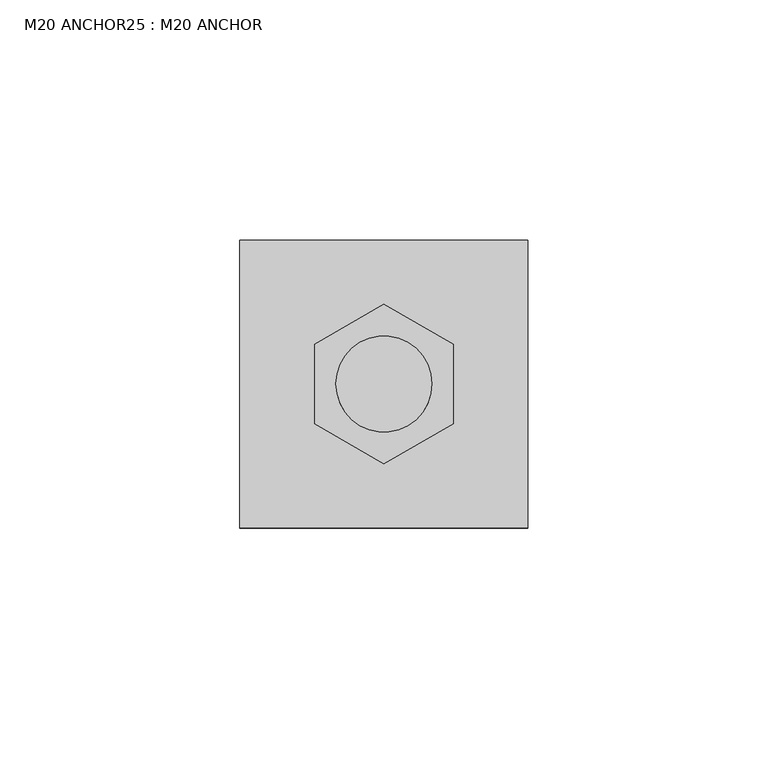
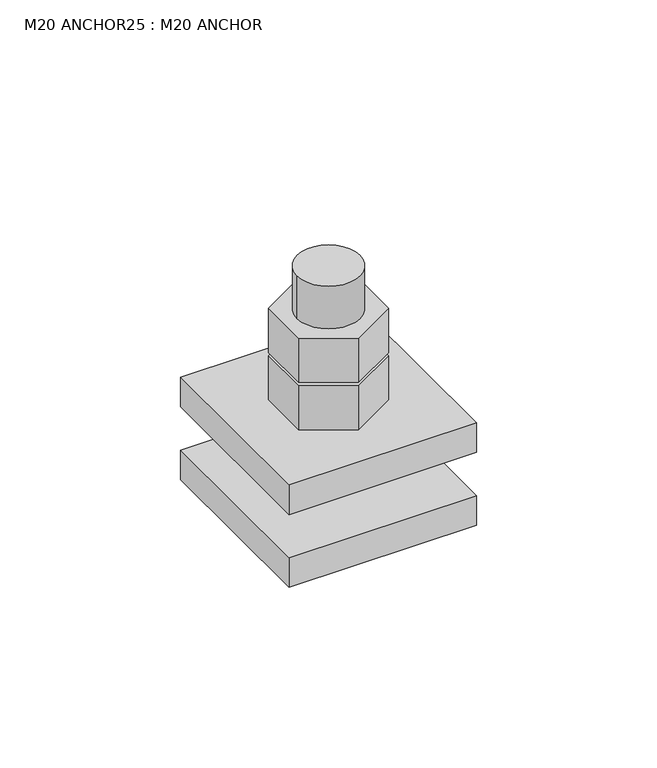
"""IFC4 building model written with IfcOpenShell, lengths in millimetres: fastener geometry, M20 ANCHOR25 : M20 ANCHOR."""

import ifcopenshell
import ifcopenshell.guid

model = None  # the IFC model being written
_history = None  # IfcOwnerHistory: only IFC2X3 demands one
_inside = {}  # id of a spatial element -> (the spatial element, [elements in it])
_under = {}  # id of a project, library or spatial element -> (it, [spatial elements below it])
_declared = {}  # id of a project -> (the project, [libraries it declares])
_typed = {}  # id of a type object -> (the type object, [elements of that type])
_made_of = {}  # id of a material, layer set ... -> (it, [elements and type objects made of it])


def new_model(schema):
    """Start an empty IFC model of exactly this schema.

    Asked for "IFC4X3", IfcOpenShell would pick the latest addendum, in which some entities
    have other attributes; the version numbers below select the first issue.
    IFC2X3 requires an IfcOwnerHistory on every rooted entity: one is made here for all.
    """
    global model, _history
    if schema == "IFC4X3":
        model = ifcopenshell.file(schema_version=(4, 3, 0, 0))
    else:
        model = ifcopenshell.file(schema=schema)
    _inside.clear()
    _under.clear()
    _declared.clear()
    _typed.clear()
    _made_of.clear()
    _history = None
    if model.schema == "IFC2X3":
        org = make("IfcOrganization", Name="unknown")
        user = make(
            "IfcPersonAndOrganization",
            ThePerson=make("IfcPerson", FamilyName="unknown"),
            TheOrganization=org,
        )
        app = make(
            "IfcApplication",
            ApplicationDeveloper=org,
            Version="unknown",
            ApplicationFullName="unknown",
            ApplicationIdentifier="unknown",
        )
        _history = make(
            "IfcOwnerHistory",
            OwningUser=user,
            OwningApplication=app,
            ChangeAction="ADDED",
            CreationDate=0,
        )
    return model


def make(cls, **values):
    """One entity of the class cls with the attributes given. An attribute that is None is left unset."""
    return model.create_entity(
        cls, **{name: value for name, value in values.items() if value is not None}
    )


def rooted(cls, **values):
    """An entity with a GlobalId (a new one), such as an element, a storey or a relation."""
    return make(cls, GlobalId=ifcopenshell.guid.new(), OwnerHistory=_history, **values)


def si_unit(unit_type, name, prefix=None):
    """IfcSIUnit, for example si_unit("LENGTHUNIT", "METRE", prefix="MILLI")."""
    return make("IfcSIUnit", UnitType=unit_type, Prefix=prefix, Name=name)


def assignment(units):
    """IfcUnitAssignment: the units of a project."""
    return None if units is None else make("IfcUnitAssignment", Units=units)


def point(xyz):
    """IfcCartesianPoint."""
    return None if xyz is None else make("IfcCartesianPoint", Coordinates=xyz)


def direction(xyz):
    """IfcDirection."""
    return None if xyz is None else make("IfcDirection", DirectionRatios=xyz)


def frame(location, z_axis=None, x_axis=None):
    """IfcAxis2Placement3D, a coordinate frame: its origin and axes. An axis left out is left unset."""
    return make(
        "IfcAxis2Placement3D",
        Location=point(location),
        Axis=direction(z_axis),
        RefDirection=direction(x_axis),
    )


def frame_2d(location, x_axis=None):
    """IfcAxis2Placement2D, a coordinate frame in the plane: its origin and x axis."""
    return make(
        "IfcAxis2Placement2D", Location=point(location), RefDirection=direction(x_axis)
    )


def origin():
    """The frame at (0, 0, 0) with its axes left unset."""
    return frame((0.0, 0.0, 0.0))


def place(relative_to, where):
    """IfcLocalPlacement: puts the frame where relative to a parent placement (None: the world)."""
    return make(
        "IfcLocalPlacement", PlacementRelTo=relative_to, RelativePlacement=where
    )


def context(
    kind, dimensions, precision=None, world=None, true_north=None, identifier=None
):
    """IfcGeometricRepresentationContext, for example the 3D "Model" context."""
    return make(
        "IfcGeometricRepresentationContext",
        ContextIdentifier=identifier,
        ContextType=kind,
        CoordinateSpaceDimension=dimensions,
        Precision=precision,
        WorldCoordinateSystem=world,
        TrueNorth=true_north,
    )


def project(units=None, contexts=None):
    """IfcProject with its units and contexts."""
    return rooted(
        "IfcProject",
        Name="project",
        RepresentationContexts=contexts,
        UnitsInContext=assignment(units),
    )


def spatial(cls, under=None, at=None, **own):
    """A site, building, storey or space (cls), placed at a placement, below another one or the project."""
    s = rooted(cls, ObjectPlacement=at, **own)
    if under is not None:
        _under.setdefault(under.id(), (under, []))[1].append(s)
    return s


def polyline(points):
    """IfcPolyline through the points."""
    return make("IfcPolyline", Points=[point(p) for p in points])


def circle_curve(where, radius):
    """IfcCircle in the frame where."""
    return make("IfcCircle", Position=where, Radius=radius)


def trimmed(basis, trim1, trim2, sense, master):
    """IfcTrimmedCurve: the piece of a basis curve between two trims."""
    return make(
        "IfcTrimmedCurve",
        BasisCurve=basis,
        Trim1=trim1,
        Trim2=trim2,
        SenseAgreement=sense,
        MasterRepresentation=master,
    )


def segment(curve, same_sense, transition):
    """IfcCompositeCurveSegment."""
    return make(
        "IfcCompositeCurveSegment",
        Transition=transition,
        SameSense=same_sense,
        ParentCurve=curve,
    )


def composite_curve(segments, self_intersect=None):
    """IfcCompositeCurve: segments joined end to end."""
    return make("IfcCompositeCurve", Segments=segments, SelfIntersect=self_intersect)


def outline(outer, holes=None, kind="AREA"):
    """IfcArbitraryClosedProfileDef: a profile drawn as a closed curve; with holes, ...WithVoids."""
    if holes is None:
        return make("IfcArbitraryClosedProfileDef", ProfileType=kind, OuterCurve=outer)
    return make(
        "IfcArbitraryProfileDefWithVoids",
        ProfileType=kind,
        OuterCurve=outer,
        InnerCurves=holes,
    )


def extrude(swept, where, along, depth):
    """IfcExtrudedAreaSolid: the profile swept, set in the frame where, extruded along a direction by depth."""
    return make(
        "IfcExtrudedAreaSolid",
        SweptArea=swept,
        Position=where,
        ExtrudedDirection=direction(along),
        Depth=depth,
    )


def shape(context_of_items, identifier, shape_type, items):
    """IfcShapeRepresentation: the items that make up one representation, for example the "Body"."""
    return make(
        "IfcShapeRepresentation",
        ContextOfItems=context_of_items,
        RepresentationIdentifier=identifier,
        RepresentationType=shape_type,
        Items=items,
    )


def source(mapping_origin, context_of_items, identifier, shape_type, items):
    """IfcRepresentationMap: a shape defined once, which mapped items show again and again."""
    return make(
        "IfcRepresentationMap",
        MappingOrigin=mapping_origin,
        MappedRepresentation=shape(context_of_items, identifier, shape_type, items),
    )


def transform(
    local_origin,
    x_axis=None,
    y_axis=None,
    z_axis=None,
    scale=None,
    scale2=None,
    scale3=None,
    uniform=True,
):
    """IfcCartesianTransformationOperator3D, or its non-uniform kind. x_axis, y_axis, z_axis: its Axis1, 2, 3."""
    if uniform:
        return make(
            "IfcCartesianTransformationOperator3D",
            Axis1=direction(x_axis),
            Axis2=direction(y_axis),
            LocalOrigin=point(local_origin),
            Scale=scale,
            Axis3=direction(z_axis),
        )
    return make(
        "IfcCartesianTransformationOperator3DnonUniform",
        Axis1=direction(x_axis),
        Axis2=direction(y_axis),
        LocalOrigin=point(local_origin),
        Scale=scale,
        Axis3=direction(z_axis),
        Scale2=scale2,
        Scale3=scale3,
    )


def mapped(mapping_source, mapping_target):
    """IfcMappedItem: shows the shape of a source again, moved by a transform."""
    return make(
        "IfcMappedItem", MappingSource=mapping_source, MappingTarget=mapping_target
    )


def made_of(thing, what):
    """Note that an element or type object is made of a material, layer set ...; save() writes the relation."""
    if what is not None:
        _made_of.setdefault(what.id(), (what, []))[1].append(thing)
    return thing


def element(
    cls,
    number,
    at=None,
    inside=None,
    cuts=None,
    type_object=None,
    material=None,
    context=None,
    identifier="Body",
    shape_type=None,
    held_by="IfcProductDefinitionShape",
    body=None,
    shapes=None,
    **own,
):
    """One element of the class cls, such as IfcWall. Its Tag is "e" and its number.

    at: its placement. inside: the storey or other place that contains it. cuts: it is an
    opening in that element (IfcRelVoidsElement). A single representation is given by context,
    identifier, shape_type and body (its items); several are given by shapes. held_by: the class
    of the entity that holds the representations. save() writes the other relations.
    """
    e = rooted(cls, Tag="e%d" % number, ObjectPlacement=at, **own)
    if body is not None:
        shapes = [shape(context, identifier, shape_type, body)]
    if shapes is not None:
        e.Representation = make(held_by, Representations=shapes)
    if inside is not None:
        _inside.setdefault(inside.id(), (inside, []))[1].append(e)
    if cuts is not None:
        rooted(
            "IfcRelVoidsElement", RelatingBuildingElement=cuts, RelatedOpeningElement=e
        )
    if type_object is not None:
        _typed.setdefault(type_object.id(), (type_object, []))[1].append(e)
    return made_of(e, material)


def aggregate(whole, parts):
    """IfcRelAggregates: a whole, such as a stair, and the parts it consists of."""
    return rooted("IfcRelAggregates", RelatingObject=whole, RelatedObjects=parts)


def save(model, path):
    """Write the relations noted so far, then the file.

    IfcRelAggregates (storeys below a building ...), IfcRelContainedInSpatialStructure (elements
    in a storey), IfcRelDefinesByType, IfcRelAssociatesMaterial and IfcRelDeclares: one each for
    every whole, place, type object, material and project.
    """
    for whole, parts in _under.values():
        aggregate(whole, parts)
    for where, things in _inside.values():
        rooted(
            "IfcRelContainedInSpatialStructure",
            RelatedElements=things,
            RelatingStructure=where,
        )
    for kind, things in _typed.values():
        rooted("IfcRelDefinesByType", RelatedObjects=things, RelatingType=kind)
    for what, things in _made_of.values():
        rooted("IfcRelAssociatesMaterial", RelatedObjects=things, RelatingMaterial=what)
    for by, libraries in _declared.values():
        rooted("IfcRelDeclares", RelatingContext=by, RelatedDefinitions=libraries)
    model.write(path)


def m20_anchor25_m20_anchor_22db5d31(model_context):
    return source(origin(), model_context, "Body", "SweptSolid", [
        extrude(outline(polyline([(-30872.0439916, -7533.2988347), (-30886.4521106, -7541.6173661), (-30900.8602297, -7533.2988347), (-30900.8602297, -7516.6617719), (-30886.4521106, -7508.3432405), (-30872.0439916, -7516.6617719), (-30872.0439916, -7533.2988347)]), holes=[composite_curve([segment(trimmed(circle_curve(frame_2d((-30886.4521106, -7524.9803033)), 10.0), [point((-30896.4521106, -7524.9803033))], [point((-30876.4521106, -7524.9803033))], True, "CARTESIAN"), True, "CONTINUOUS"), segment(trimmed(circle_curve(frame_2d((-30886.4521106, -7524.9803033)), 10.0), [point((-30876.4521106, -7524.9803033))], [point((-30896.4521106, -7524.9803033))], True, "CARTESIAN"), True, "CONTINUOUS")], self_intersect=False)]), frame((0.0, 0.0, 240.6), z_axis=(0.0, 0.0, 1.0), x_axis=(1.0, 0.0, 0.0)), (0.0, 0.0, 1.0), 15.0),
        extrude(outline(polyline([(-30872.0439916, -7533.2988347), (-30886.4521106, -7541.6173661), (-30900.8602297, -7533.2988347), (-30900.8602297, -7516.6617719), (-30886.4521106, -7508.3432405), (-30872.0439916, -7516.6617719), (-30872.0439916, -7533.2988347)]), holes=[composite_curve([segment(trimmed(circle_curve(frame_2d((-30886.4521106, -7524.9803033)), 10.0), [point((-30896.4521106, -7524.9803033))], [point((-30876.4521106, -7524.9803033))], True, "CARTESIAN"), True, "CONTINUOUS"), segment(trimmed(circle_curve(frame_2d((-30886.4521106, -7524.9803033)), 10.0), [point((-30876.4521106, -7524.9803033))], [point((-30896.4521106, -7524.9803033))], True, "CARTESIAN"), True, "CONTINUOUS")], self_intersect=False)]), frame((0.0, 0.0, 224.6), z_axis=(0.0, 0.0, 1.0), x_axis=(1.0, 0.0, 0.0)), (0.0, 0.0, 1.0), 15.0),
        extrude(outline(composite_curve([segment(trimmed(circle_curve(frame_2d((-30886.4521106, -7524.9803033)), 10.0), [point((-30896.4521106, -7524.9803033))], [point((-30876.4521106, -7524.9803033))], False, "CARTESIAN"), True, "CONTINUOUS"), segment(trimmed(circle_curve(frame_2d((-30886.4521106, -7524.9803033)), 10.0), [point((-30876.4521106, -7524.9803033))], [point((-30896.4521106, -7524.9803033))], False, "CARTESIAN"), True, "CONTINUOUS")], self_intersect=False)), frame((0.0, 0.0, 190.0), z_axis=(0.0, 0.0, 1.0), x_axis=(1.0, 0.0, 0.0)), (0.0, 0.0, 1.0), 80.0),
        extrude(outline(polyline([(-30856.4521106, -7554.9803033), (-30916.4521106, -7554.9803033), (-30916.4521106, -7494.9803033), (-30856.4521106, -7494.9803033), (-30856.4521106, -7554.9803033)]), holes=[composite_curve([segment(trimmed(circle_curve(frame_2d((-30886.4521106, -7524.9803033)), 11.0), [point((-30897.4521106, -7524.9803033))], [point((-30875.4521106, -7524.9803033))], True, "CARTESIAN"), True, "CONTINUOUS"), segment(trimmed(circle_curve(frame_2d((-30886.4521106, -7524.9803033)), 11.0), [point((-30875.4521106, -7524.9803033))], [point((-30897.4521106, -7524.9803033))], True, "CARTESIAN"), True, "CONTINUOUS")], self_intersect=False)]), frame((0.0, 0.0, 190.0), z_axis=(0.0, 0.0, 1.0), x_axis=(1.0, 0.0, 0.0)), (0.0, 0.0, 1.0), 10.0),
        extrude(outline(polyline([(-30856.4521106, -7554.9803033), (-30916.4521106, -7554.9803033), (-30916.4521106, -7494.9803033), (-30856.4521106, -7494.9803033), (-30856.4521106, -7554.9803033)]), holes=[composite_curve([segment(trimmed(circle_curve(frame_2d((-30886.4521106, -7524.9803033)), 11.0), [point((-30897.4521106, -7524.9803033))], [point((-30875.4521106, -7524.9803033))], True, "CARTESIAN"), True, "CONTINUOUS"), segment(trimmed(circle_curve(frame_2d((-30886.4521106, -7524.9803033)), 11.0), [point((-30875.4521106, -7524.9803033))], [point((-30897.4521106, -7524.9803033))], True, "CARTESIAN"), True, "CONTINUOUS")], self_intersect=False)]), frame((0.0, 0.0, 214.6), z_axis=(0.0, 0.0, 1.0), x_axis=(1.0, 0.0, 0.0)), (0.0, 0.0, 1.0), 10.0),
    ])


if __name__ == "__main__":
    model = new_model("IFC4")
    model_context = context("Model", 3, world=origin())
    ifc_project = project(units=[si_unit("LENGTHUNIT", "METRE", prefix="MILLI")], contexts=[model_context])
    site = spatial("IfcSite", under=ifc_project)
    building = spatial("IfcBuilding", under=site)
    placement = place(None, origin())
    m20_anchor25_m20_anchor_shape = m20_anchor25_m20_anchor_22db5d31(model_context)
    element("IfcFastener", 1, ObjectType="M20 ANCHOR25 : M20 ANCHOR", at=placement, inside=building, context=model_context, shape_type="MappedRepresentation", body=[
        mapped(m20_anchor25_m20_anchor_shape, transform((0.0, 0.0, 0.0), x_axis=(1.0, 0.0, 0.0), y_axis=(0.0, 1.0, 0.0), z_axis=(0.0, 0.0, 1.0))),
    ])
    save(model, "model.ifc")
